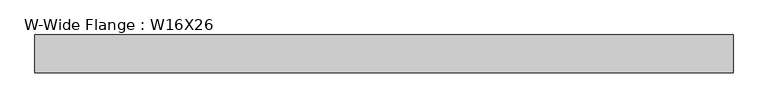
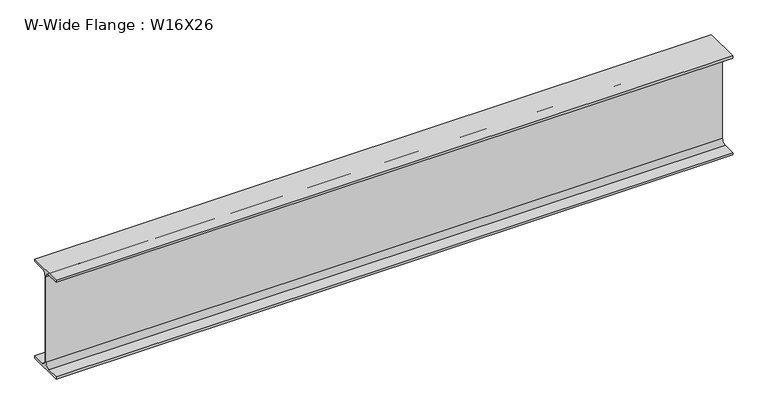
"""IFC4 building model written with IfcOpenShell, lengths in millimetres: beam geometry, W-Wide Flange : W16X26."""

from ifc_helpers import new_model, si_unit, point, frame, frame_2d, origin, place, context, project, spatial, polyline, circle_curve, trimmed, segment, composite_curve, outline, extrude, source, transform, mapped, element, save


def w_wide_flange_w16x26_f2924dd3(model_context):
    return source(origin(), model_context, "Body", "SweptSolid", [
        extrude(outline(composite_curve([segment(polyline([(69.85, -190.627), (69.85, -199.39), (-69.85, -199.39), (-69.85, -190.627), (-21.3995, -190.627)]), True, "CONTINUOUS"), segment(trimmed(circle_curve(frame_2d((-21.3995, -172.4025)), 18.2245), [point((-21.3995, -190.627))], [point((-3.175, -172.4025))], True, "CARTESIAN"), True, "CONTINUOUS"), segment(polyline([(-3.175, -172.4025), (-3.175, 172.4025)]), True, "CONTINUOUS"), segment(trimmed(circle_curve(frame_2d((-21.3995, 172.4025)), 18.2245), [point((-3.175, 172.4025))], [point((-21.3995, 190.627))], True, "CARTESIAN"), True, "CONTINUOUS"), segment(polyline([(-21.3995, 190.627), (-69.85, 190.627), (-69.85, 199.39), (69.85, 199.39), (69.85, 190.627), (21.3995, 190.627)]), True, "CONTINUOUS"), segment(trimmed(circle_curve(frame_2d((21.3995, 172.4025)), 18.2245), [point((21.3995, 190.627))], [point((3.175, 172.4025))], True, "CARTESIAN"), True, "CONTINUOUS"), segment(polyline([(3.175, 172.4025), (3.175, -172.4025)]), True, "CONTINUOUS"), segment(trimmed(circle_curve(frame_2d((21.3995, -172.4025)), 18.2245), [point((3.175, -172.4025))], [point((21.3995, -190.627))], True, "CARTESIAN"), True, "CONTINUOUS"), segment(polyline([(21.3995, -190.627), (69.85, -190.627)]), True, "CONTINUOUS")], self_intersect=False)), frame((-1298.2637019, 0.0, 0.0), z_axis=(1.0, 0.0, 0.0), x_axis=(0.0, 1.0, 0.0)), (0.0, 0.0, 1.0), 2582.1439446),
    ])


if __name__ == "__main__":
    model = new_model("IFC4")
    model_context = context("Model", 3, world=origin())
    ifc_project = project(units=[si_unit("LENGTHUNIT", "METRE", prefix="MILLI")], contexts=[model_context])
    site = spatial("IfcSite", under=ifc_project)
    building = spatial("IfcBuilding", under=site)
    placement = place(None, origin())
    w_wide_flange_w16x26_shape = w_wide_flange_w16x26_f2924dd3(model_context)
    element("IfcBeam", 1, ObjectType="W-Wide Flange : W16X26", at=placement, inside=building, context=model_context, shape_type="MappedRepresentation", body=[
        mapped(w_wide_flange_w16x26_shape, transform((0.0, 0.0, 0.0), x_axis=(1.0, 0.0, 0.0), y_axis=(0.0, 1.0, 0.0), z_axis=(0.0, 0.0, 1.0))),
    ])
    save(model, "model.ifc")

# Revit data of these elements
# Type "W-Wide Flange : W16X26"
#   Assembly Code = "B10"
#   W = 26
#   Length [instance default] = 5' - 0"
#   bf = 0' - 5 1/2"
#   d = 1' - 3.7"
#   k = 0' - 1 1/16"
#   k2 = 0' - 0.7175"
#   tf = 0' - 0.345"
#   tw = 0' - 0 1/4"
#   A = 0.0533333 SF
#   Structural Material [instance default] = Steel ASTM A992
# Element 1 (IfcBeam, "W-Wide Flange : W16X26")
#   Structural Material = Steel ASTM A36
#   Materials on its faces: "Steel ASTM A36"
# Materials
#   "Steel ASTM A992": class "Metal", colour RGB 199 199 199, transparency 0, Description = "Structural steel 50ksi", Cost = 0
#   "Steel ASTM A36": class "Metal", colour RGB 199 199 199, transparency 0, Description = "Structural steel, ASTM A36 Grade B, mill finish", Cost = 0
